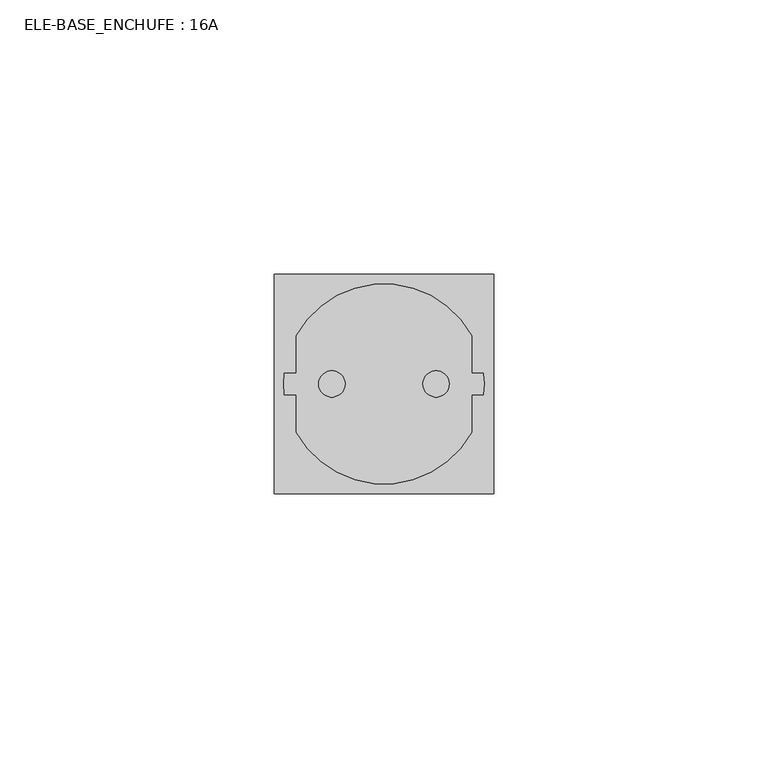
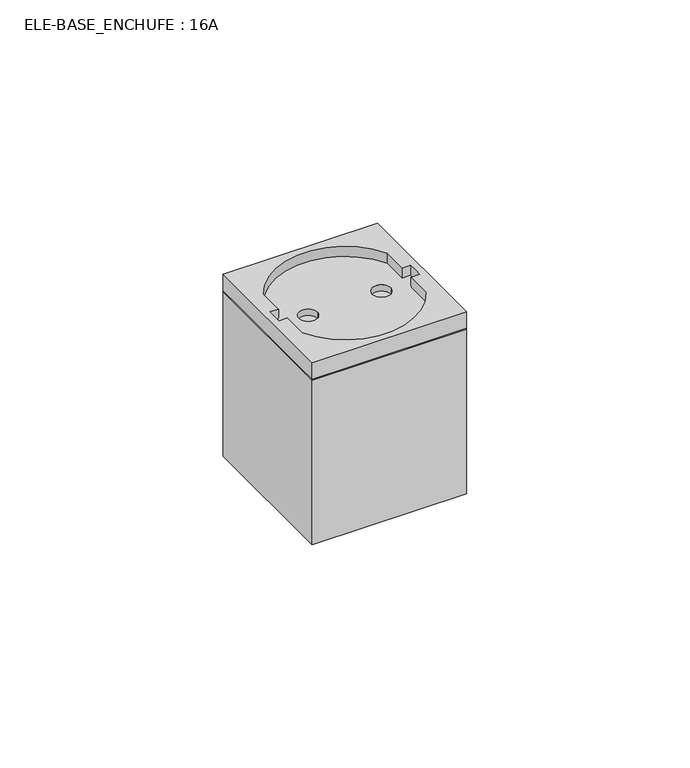
"""IFC4 building model written with IfcOpenShell, lengths in millimetres: proxy geometry, ELE-BASE_ENCHUFE : 16A."""

from ifc_helpers import new_model, si_unit, frame, origin, place, context, project, spatial, polyline, circle_curve, outline, extrude, source, transform, mapped, element, save
from ifc_brep_helpers import plane_surface, revolved_surface, advanced_brep


def ele_base_enchufe_16a_49acce93(model_context):
    return source(origin(), model_context, "Body", "SolidModel", [
        extrude(outline(polyline([(20.0, -20.0), (-20.0, -20.0), (-20.0, 20.0), (20.0, 20.0), (20.0, -20.0)])), frame((0.0, 0.0, -45.0), z_axis=(0.0, 0.0, 1.0), x_axis=(1.0, 0.0, 0.0)), (0.0, 0.0, 1.0), 45.0),
        advanced_brep(
        [(20.0, -20.0, 4.7625), (20.0, 20.0, 4.7625), (-20.0, 20.0, 4.7625), (-20.0, -20.0, 4.7625), (-16.0, 8.7785249, 4.7625), (16.0, 8.7785249, 4.7625), (16.0, 2.0, 4.7625), (18.1400799, 2.0, 4.7625), (18.1400799, -2.0, 4.7625), (16.0, -2.0, 4.7625), (16.0, -8.7785249, 4.7625), (-16.0, -8.7785249, 4.7625), (-16.0, -2.0, 4.7625), (-18.1400799, -2.0, 4.7625), (-18.1400799, 2.0, 4.7625), (-16.0, 2.0, 4.7625), (20.0, -20.0, 0.0), (-20.0, -20.0, 0.0), (-20.0, 20.0, 0.0), (20.0, 20.0, 0.0), (-11.9, 0.0, 0.0), (-7.1, 0.0, 0.0), (7.1, 0.0, 0.0), (11.9, 0.0, 0.0), (-16.0, 2.0, 2.0), (-18.1400799, 2.0, 2.0), (-18.1400799, -2.0, 2.0), (-16.0, -2.0, 2.0), (-16.0, -8.7785249, 2.0), (16.0, -8.7785249, 2.0), (16.0, -2.0, 2.0), (18.1400799, -2.0, 2.0), (18.1400799, 2.0, 2.0), (16.0, 2.0, 2.0), (16.0, 8.7785249, 2.0), (-16.0, 8.7785249, 2.0), (-7.1, 0.0, 2.0), (-11.9, 0.0, 2.0), (11.9, 0.0, 2.0), (7.1, 0.0, 2.0)],
        [
            (0, 1),
            (1, 2),
            (2, 3),
            (3, 0),
            (4, 5, circle_curve(frame((0.0, 0.0, 4.7625), z_axis=(0.0, 0.0, -1.0), x_axis=(1.0, 0.0, 0.0)), 18.25)),
            (5, 6),
            (6, 7),
            (7, 8, circle_curve(frame((0.0, 0.0, 4.7625), z_axis=(0.0, 0.0, -1.0), x_axis=(1.0, 0.0, 0.0)), 18.25)),
            (8, 9),
            (9, 10),
            (10, 11, circle_curve(frame((0.0, 0.0, 4.7625), z_axis=(0.0, 0.0, -1.0), x_axis=(1.0, 0.0, 0.0)), 18.25)),
            (11, 12),
            (12, 13),
            (13, 14, circle_curve(frame((0.0, 0.0, 4.7625), z_axis=(0.0, 0.0, -1.0), x_axis=(1.0, 0.0, 0.0)), 18.25)),
            (14, 15),
            (15, 4),
            (16, 17),
            (17, 18),
            (18, 19),
            (19, 16),
            (20, 21, circle_curve(frame((-9.5, 0.0, 0.0), z_axis=(0.0, 0.0, 1.0), x_axis=(1.0, 0.0, 0.0)), 2.4)),
            (21, 20, circle_curve(frame((-9.5, 0.0, 0.0), z_axis=(0.0, 0.0, 1.0), x_axis=(1.0, 0.0, 0.0)), 2.4)),
            (22, 23, circle_curve(frame((9.5, 0.0, 0.0), z_axis=(0.0, 0.0, 1.0), x_axis=(1.0, 0.0, 0.0)), 2.4)),
            (23, 22, circle_curve(frame((9.5, 0.0, 0.0), z_axis=(0.0, 0.0, 1.0), x_axis=(1.0, 0.0, 0.0)), 2.4)),
            (3, 17),
            (16, 0),
            (2, 18),
            (1, 19),
            (24, 25),
            (25, 26, circle_curve(frame((0.0, 0.0, 2.0), z_axis=(0.0, 0.0, 1.0), x_axis=(1.0, 0.0, 0.0)), 18.25)),
            (26, 27),
            (27, 28),
            (28, 29, circle_curve(frame((0.0, 0.0, 2.0), z_axis=(0.0, 0.0, 1.0), x_axis=(1.0, 0.0, 0.0)), 18.25)),
            (29, 30),
            (30, 31),
            (31, 32, circle_curve(frame((0.0, 0.0, 2.0), z_axis=(0.0, 0.0, 1.0), x_axis=(1.0, 0.0, 0.0)), 18.25)),
            (32, 33),
            (33, 34),
            (34, 35, circle_curve(frame((0.0, 0.0, 2.0), z_axis=(0.0, 0.0, 1.0), x_axis=(1.0, 0.0, 0.0)), 18.25)),
            (35, 24),
            (36, 37, circle_curve(frame((-9.5, 0.0, 2.0), z_axis=(0.0, 0.0, -1.0), x_axis=(1.0, 0.0, 0.0)), 2.4)),
            (37, 36, circle_curve(frame((-9.5, 0.0, 2.0), z_axis=(0.0, 0.0, -1.0), x_axis=(1.0, 0.0, 0.0)), 2.4)),
            (38, 39, circle_curve(frame((9.5, 0.0, 2.0), z_axis=(0.0, 0.0, -1.0), x_axis=(1.0, 0.0, 0.0)), 2.4)),
            (39, 38, circle_curve(frame((9.5, 0.0, 2.0), z_axis=(0.0, 0.0, -1.0), x_axis=(1.0, 0.0, 0.0)), 2.4)),
            (35, 4),
            (15, 24),
            (34, 5),
            (33, 6),
            (32, 7),
            (31, 8),
            (30, 9),
            (29, 10),
            (28, 11),
            (27, 12),
            (26, 13),
            (25, 14),
            (21, 36),
            (37, 20),
            (23, 38),
            (39, 22),
        ],
        [
            plane_surface(frame((-40.0, -20.0, 4.7625), z_axis=(0.0, 0.0, 1.0), x_axis=(-1.0, 0.0, 0.0))),
            plane_surface(frame((-40.0, -20.0, 0.0), z_axis=(0.0, 0.0, -1.0), x_axis=(1.0, 0.0, 0.0))),
            plane_surface(frame((20.0, -20.0, 4.7625), z_axis=(0.0, -1.0, 0.0), x_axis=(0.0, 0.0, -1.0))),
            plane_surface(frame((-20.0, -20.0, 4.7625), z_axis=(-1.0, 0.0, 0.0), x_axis=(0.0, 0.0, -1.0))),
            plane_surface(frame((-20.0, 20.0, 4.7625), z_axis=(0.0, 1.0, 0.0), x_axis=(0.0, 0.0, -1.0))),
            plane_surface(frame((20.0, 20.0, 4.7625), z_axis=(1.0, 0.0, 0.0), x_axis=(0.0, 0.0, -1.0))),
            plane_surface(frame((-16.0, 8.7785249, 2.0), z_axis=(0.0, 0.0, 1.0), x_axis=(0.0, -1.0, 0.0))),
            plane_surface(frame((-16.0, 2.0, 4.8), z_axis=(1.0, 0.0, 0.0), x_axis=(0.0, 0.0, -1.0))),
            revolved_surface(polyline([(18.25, 0.0, 4.7625), (18.25, 0.0, 2.0)]), (0.0, 0.0, 2.0), (0.0, 0.0, 1.0)),
            plane_surface(frame((16.0, 8.7785249, 4.8), z_axis=(-1.0, 0.0, 0.0), x_axis=(0.0, 0.0, -1.0))),
            plane_surface(frame((16.0, 2.0, 4.8), z_axis=(0.0, -1.0, 0.0), x_axis=(0.0, 0.0, -1.0))),
            plane_surface(frame((18.1400799, -2.0, 4.8), z_axis=(0.0, 1.0, 0.0), x_axis=(0.0, 0.0, -1.0))),
            plane_surface(frame((16.0, -2.0, 4.8), z_axis=(-1.0, 0.0, 0.0), x_axis=(0.0, 0.0, -1.0))),
            plane_surface(frame((-16.0, -8.7785249, 4.8), z_axis=(1.0, 0.0, 0.0), x_axis=(0.0, 0.0, -1.0))),
            plane_surface(frame((-16.0, -2.0, 4.8), z_axis=(0.0, 1.0, 0.0), x_axis=(0.0, 0.0, -1.0))),
            plane_surface(frame((-18.1400799, 2.0, 4.8), z_axis=(0.0, -1.0, 0.0), x_axis=(0.0, 0.0, -1.0))),
            revolved_surface(polyline([(-7.1, 0.0, 2.0), (-7.1, 0.0, 0.0)]), (-9.5, 0.0, -18.0), (0.0, 0.0, 1.0)),
            revolved_surface(polyline([(11.9, 0.0, 2.0), (11.9, 0.0, 0.0)]), (9.5, 0.0, 0.0), (0.0, 0.0, 1.0)),
        ],
        [
            (0, [[1, 2, 3, 4], [5, 6, 7, 8, 9, 10, 11, 12, 13, 14, 15, 16]]),
            (1, [[17, 18, 19, 20], [21, 22], [23, 24]]),
            (2, [[25, -17, 26, -4]]),
            (3, [[27, -18, -25, -3]]),
            (4, [[28, -19, -27, -2]]),
            (5, [[-26, -20, -28, -1]]),
            (6, [[29, 30, 31, 32, 33, 34, 35, 36, 37, 38, 39, 40], [41, 42], [43, 44]]),
            (7, [[45, -16, 46, -40]]),
            (8, [[47, -5, -45, -39]]),
            (9, [[48, -6, -47, -38]]),
            (10, [[49, -7, -48, -37]]),
            (8, [[50, -8, -49, -36]]),
            (11, [[51, -9, -50, -35]]),
            (12, [[52, -10, -51, -34]]),
            (8, [[53, -11, -52, -33]]),
            (13, [[54, -12, -53, -32]]),
            (14, [[55, -13, -54, -31]]),
            (8, [[56, -14, -55, -30]]),
            (15, [[-46, -15, -56, -29]]),
            (16, [[-22, 57, -42, 58]]),
            (16, [[-41, -57, -21, -58]]),
            (17, [[-24, 59, -44, 60]]),
            (17, [[-43, -59, -23, -60]]),
        ],
    ),
    ])


if __name__ == "__main__":
    model = new_model("IFC4")
    model_context = context("Model", 3, world=origin())
    ifc_project = project(units=[si_unit("LENGTHUNIT", "METRE", prefix="MILLI")], contexts=[model_context])
    site = spatial("IfcSite", under=ifc_project)
    building = spatial("IfcBuilding", under=site)
    placement = place(None, origin())
    ele_base_enchufe_16a_shape = ele_base_enchufe_16a_49acce93(model_context)
    element("IfcBuildingElementProxy", 1, Name="ELE-BASE_ENCHUFE : 16A", ObjectType="ELE-BASE_ENCHUFE : 16A", at=placement, inside=building, context=model_context, shape_type="MappedRepresentation", body=[
        mapped(ele_base_enchufe_16a_shape, transform((0.0, 0.0, 0.0), x_axis=(1.0, 0.0, 0.0), y_axis=(0.0, 1.0, 0.0), z_axis=(0.0, 0.0, 1.0))),
    ])
    save(model, "model.ifc")

# Revit data of these elements
# Project information
#   Fecha de emisión de proyecto = "Fecha de emisión"
#   Estado de proyecto = "Estado de proyecto"
#   Nombre de cliente = "Propietario"
#   Dirección de proyecto = "Introduzca dirección aquí"
#   Nombre de proyecto = "Nombre de proyecto"
#   Número de proyecto = "0001"
# Type "ELE-BASE_ENCHUFE : 16A"
#   Etiqueta = ""
#   Voltaje toma corriente = 230 V
#   SimboloPosicionVertical [instance default] = 0.05 m
#   SimboloPosicionHorizontal [instance default] = 0.00 m
#   Potencia = 3680 W
#   Intensidad = 16 A
#   Carga = 3680 VA
#   Default Elevation = 0.20 m
#   Altura = 0.20 m
#   Simbolo25A = no
#   Simbolo16AEstanco = no
#   Simbolo16A = yes
#   Clasificación de carga = Toma de corriente
#   Assembly Code = ""
